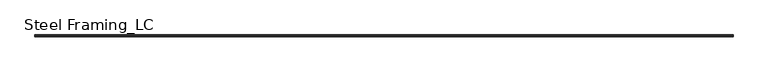
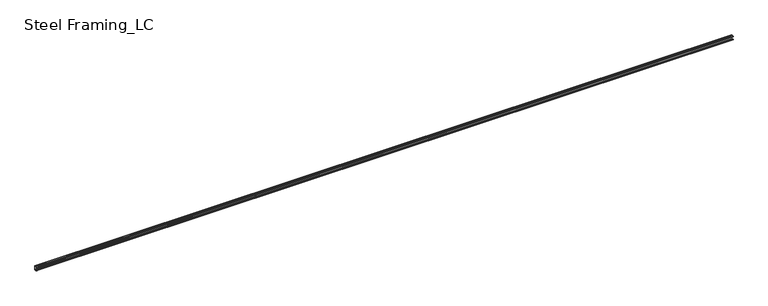
"""IFC4 building model written with IfcOpenShell, lengths in millimetres: beam geometry, Steel Framing_LC : H_SB_AR_S00_LC-150x75x25x3.2."""

from ifc_helpers import new_model, si_unit, point, frame, frame_2d, origin, place, context, project, spatial, polyline, circle_curve, trimmed, segment, composite_curve, outline, extrude, source, transform, mapped, element, save


def steel_framing_lc_f9ca99c4(model_context):
    return source(origin(), model_context, "Body", "SweptSolid", [
        extrude(outline(composite_curve([segment(polyline([(18.6, 67.0), (18.6, -67.0)]), True, "CONTINUOUS"), segment(trimmed(circle_curve(frame_2d((10.6, -67.0)), 8.0), [point((18.6, -67.0))], [point((10.6, -75.0))], False, "CARTESIAN"), True, "CONTINUOUS"), segment(polyline([(10.6, -75.0), (-48.4, -75.0)]), True, "CONTINUOUS"), segment(trimmed(circle_curve(frame_2d((-48.4, -67.0)), 8.0), [point((-48.4, -75.0))], [point((-56.4, -67.0))], False, "CARTESIAN"), True, "CONTINUOUS"), segment(polyline([(-56.4, -67.0), (-56.4, -50.0), (-53.2, -50.0), (-53.2, -67.0)]), True, "CONTINUOUS"), segment(trimmed(circle_curve(frame_2d((-48.4, -67.0)), 4.8), [point((-53.2, -67.0))], [point((-48.4, -71.8))], True, "CARTESIAN"), True, "CONTINUOUS"), segment(polyline([(-48.4, -71.8), (10.6, -71.8)]), True, "CONTINUOUS"), segment(trimmed(circle_curve(frame_2d((10.6, -67.0)), 4.8), [point((10.6, -71.8))], [point((15.4, -67.0))], True, "CARTESIAN"), True, "CONTINUOUS"), segment(polyline([(15.4, -67.0), (15.4, 67.0)]), True, "CONTINUOUS"), segment(trimmed(circle_curve(frame_2d((10.6, 67.0)), 4.8), [point((15.4, 67.0))], [point((10.6, 71.8))], True, "CARTESIAN"), True, "CONTINUOUS"), segment(polyline([(10.6, 71.8), (-48.4, 71.8)]), True, "CONTINUOUS"), segment(trimmed(circle_curve(frame_2d((-48.4, 67.0)), 4.8), [point((-48.4, 71.8))], [point((-53.2, 67.0))], True, "CARTESIAN"), True, "CONTINUOUS"), segment(polyline([(-53.2, 67.0), (-53.2, 50.0), (-56.4, 50.0), (-56.4, 67.0)]), True, "CONTINUOUS"), segment(trimmed(circle_curve(frame_2d((-48.4, 67.0)), 8.0), [point((-56.4, 67.0))], [point((-48.4, 75.0))], False, "CARTESIAN"), True, "CONTINUOUS"), segment(polyline([(-48.4, 75.0), (10.6, 75.0)]), True, "CONTINUOUS"), segment(trimmed(circle_curve(frame_2d((10.6, 67.0)), 8.0), [point((10.6, 75.0))], [point((18.6, 67.0))], False, "CARTESIAN"), True, "CONTINUOUS")], self_intersect=False)), frame((-12797.0, 0.0, 0.0), z_axis=(1.0, 0.0, 0.0), x_axis=(0.0, 1.0, 0.0)), (0.0, 0.0, 1.0), 25581.0),
    ])


if __name__ == "__main__":
    model = new_model("IFC4")
    model_context = context("Model", 3, world=origin())
    ifc_project = project(units=[si_unit("LENGTHUNIT", "METRE", prefix="MILLI")], contexts=[model_context])
    site = spatial("IfcSite", under=ifc_project)
    building = spatial("IfcBuilding", under=site)
    placement = place(None, origin())
    steel_framing_lc_shape = steel_framing_lc_f9ca99c4(model_context)
    element("IfcBeam", 1, ObjectType="Steel Framing_LC : H_SB_AR_S00_LC-150x75x25x3.2", at=placement, inside=building, context=model_context, shape_type="MappedRepresentation", body=[
        mapped(steel_framing_lc_shape, transform((0.0, 0.0, 0.0), x_axis=(1.0, 0.0, 0.0), y_axis=(0.0, 1.0, 0.0), z_axis=(0.0, 0.0, 1.0))),
    ])
    save(model, "model.ifc")

# Revit data of these elements
# Type "Steel Framing_LC : H_SB_AR_S00_LC-150x75x25x3.2"
#   Type Comments = "SECONDARY"
#   Type Mark = "GIRTH"
#   H_SectionID = "LC-150x75x25x3.2"
#   r = 4.8 mm
#   d = 25 mm
#   R = 8 mm
#   Perimeter = 0.70 m²/m
#   Nominal Weight = 10.30 kgf/m
#   Length [instance default] = 1000 mm
#   b = 75 mm
#   h = 150 mm
#   tw = 3.2 mm
#   x = 18.6 mm
#   A = 1.00 m²
#   Structural Material [instance default] = Steel, 45-345
#   Assembly Code = ""
# Element 1 (IfcBeam, "Steel Framing_LC : H_SB_AR_S00_LC-150x75x25x3.2")
#   Materials on its faces: "Steel, 45-345"
# Materials
#   "Steel, 45-345": class "Metal", colour RGB 189 187 185, transparency 0, Description = "Steel 345 MPa", Cost = 0
